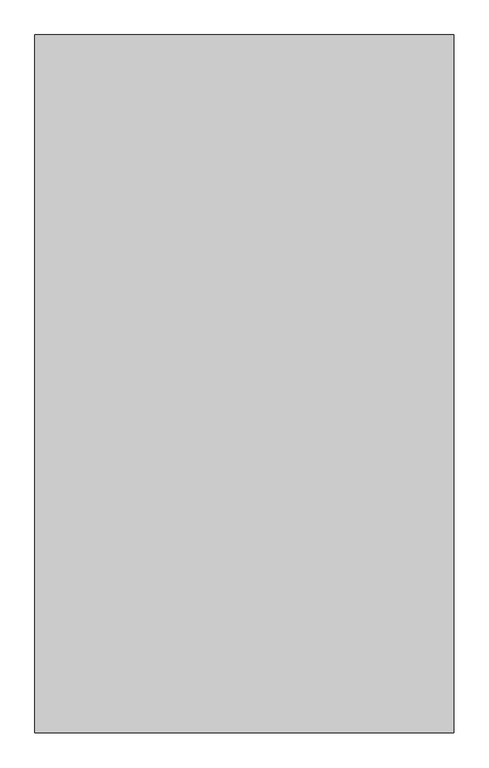
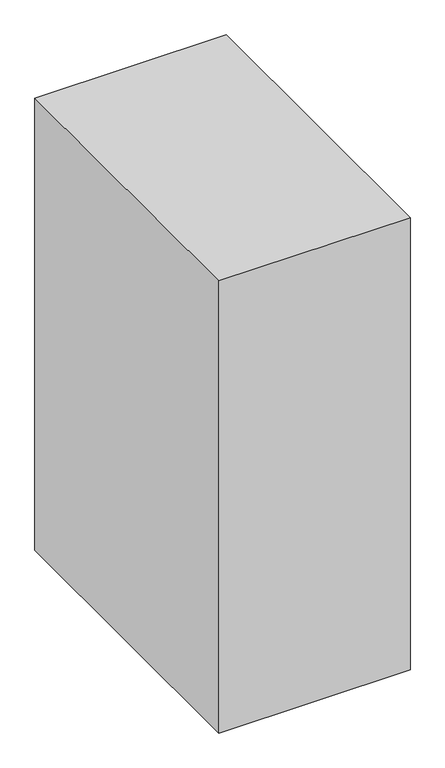
"""IFC4 building model written with IfcOpenShell, lengths in millimetres: proxy geometry, Space Planning Box_hec : Space Planning Box_hec."""

from ifc_helpers import new_model, si_unit, origin, origin_with_axes, place, context, project, spatial, polyline, outline, extrude, source, transform, mapped, element, save


def generic_models_47b98be1(model_context):
    return source(origin(), model_context, "Body", "SweptSolid", [
        extrude(outline(polyline([(1200.0, 2000.0), (1200.0, -2000.0), (-1200.0, -2000.0), (-1200.0, 2000.0), (1200.0, 2000.0)])), origin_with_axes(), (0.0, 0.0, 1.0), 6000.0),
    ])


if __name__ == "__main__":
    model = new_model("IFC4")
    model_context = context("Model", 3, world=origin())
    ifc_project = project(units=[si_unit("LENGTHUNIT", "METRE", prefix="MILLI")], contexts=[model_context])
    site = spatial("IfcSite", under=ifc_project)
    building = spatial("IfcBuilding", under=site)
    placement = place(None, origin())
    generic_models_shape = generic_models_47b98be1(model_context)
    element("IfcBuildingElementProxy", 1, Name="Space Planning Box_hec : Space Planning Box_hec", ObjectType="Space Planning Box_hec : Space Planning Box_hec", at=placement, inside=building, context=model_context, shape_type="MappedRepresentation", body=[
        mapped(generic_models_shape, transform((0.0, 0.0, 0.0), x_axis=(1.0, 0.0, 0.0), y_axis=(0.0, 1.0, 0.0), z_axis=(0.0, 0.0, 1.0))),
    ])
    save(model, "model.ifc")

# Revit data of these elements
# Type "Space Planning Box_hec : Space Planning Box_hec"
#   Type Comments = "..."
#   Room Name [instance default] = "?"
#   Interior Finish [instance default] = ""
#   Exterior Finish [instance default] = ""
#   Department [instance default] = ""
#   Assembly Code = "..."
#   Width [instance default] = 1524 mm
#   Program Area [instance default] = 0 m²
#   Length [instance default] = 1524 mm
#   Height [instance default] = 1524 mm
#   Area [instance default] = 2.32258 m²
#   Fill Color [instance default] = Cyan
#   Default Elevation = 0
# Element 1 (IfcBuildingElementProxy, "Space Planning Box_hec : Space Planning Box_hec")
#   Room Name = "Locker Room (F)"
#   Interior Finish = "IF2-1"
#   Exterior Finish = "EF1"
#   Department = "AR"
#   Width = 2400 mm
#   Program Area = 31.5 m²
#   Length = 4000 mm
#   Height = 6000 mm
#   Area = 9.6 m²
#   Fill Color = Lavender
#   Materials on its faces: "Lavender"
# Materials
#   "Cyan": class "Generic", colour RGB 0 255 255, transparency 0.2, Cost = 0
#   "Lavender": class "Generic", colour RGB 186 85 211, transparency 0.2, Cost = 0
